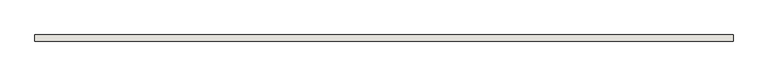
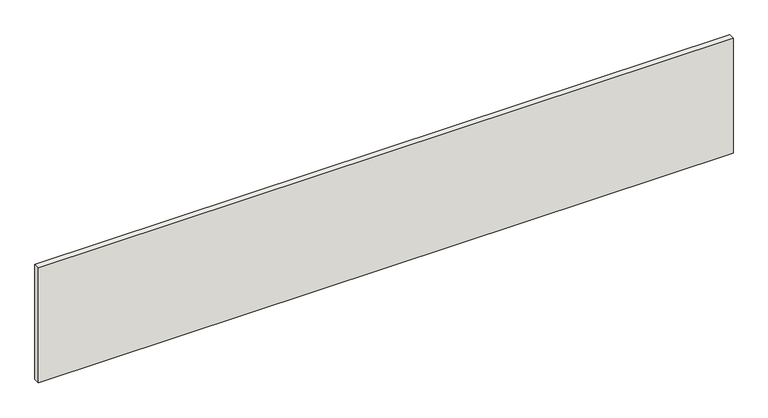
"""IFC4 building model written with IfcOpenShell, lengths in millimetres: wall geometry, 0_3d."""

from ifc_helpers import new_model, si_unit, origin, origin_with_axes, place, context, project, spatial, polyline, outline, extrude, source, transform, mapped, element, save


def wall_ee502792(model_context):
    return source(origin(), model_context, "Body", "SweptSolid", [
        extrude(outline(polyline([(0.0, 50.0), (5720.0, 50.0), (5720.0, 0.0), (0.0, 0.0), (0.0, 50.0)])), origin_with_axes(), (0.0, 0.0, 1.0), 1000.0),
    ])


if __name__ == "__main__":
    model = new_model("IFC4")
    model_context = context("Model", 3, world=origin())
    ifc_project = project(units=[si_unit("LENGTHUNIT", "METRE", prefix="MILLI")], contexts=[model_context])
    site = spatial("IfcSite", under=ifc_project)
    building = spatial("IfcBuilding", under=site)
    placement = place(None, origin())
    wall_shape = wall_ee502792(model_context)
    element("IfcWall", 1, ObjectType="0_3d", at=placement, inside=building, context=model_context, shape_type="MappedRepresentation", body=[
        mapped(wall_shape, transform((0.0, 0.0, 0.0), x_axis=(1.0, 0.0, 0.0), y_axis=(0.0, 1.0, 0.0), z_axis=(0.0, 0.0, 1.0))),
    ])
    save(model, "model.ifc")

# Revit data of these elements
# Element 1 (IfcWall, "0_3d")
#   Materials on its faces: "material wardrobe b 1"
# Materials
#   "material wardrobe b 1": class "Unassigned", colour RGB 128 128 128, transparency 0
